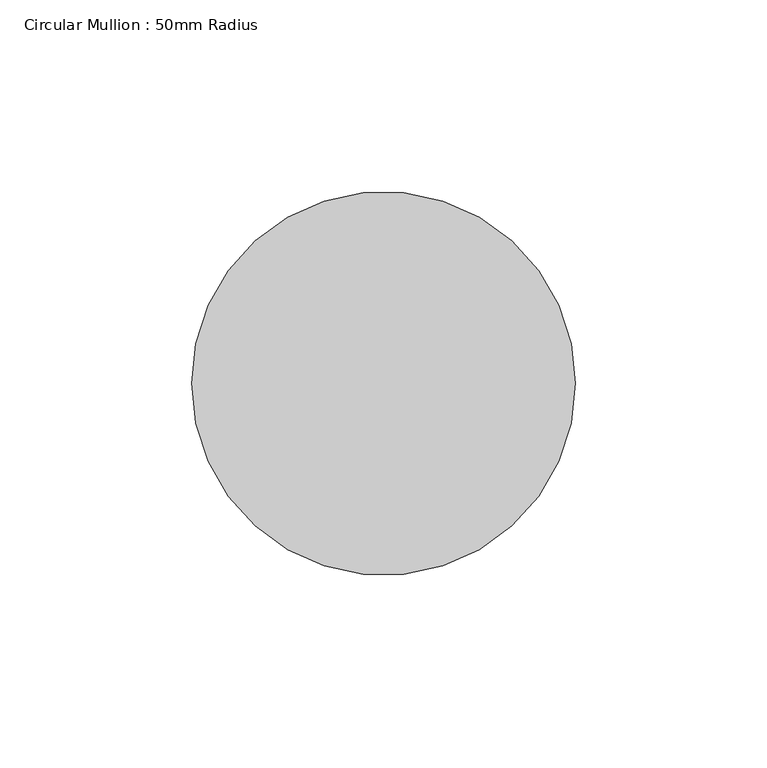
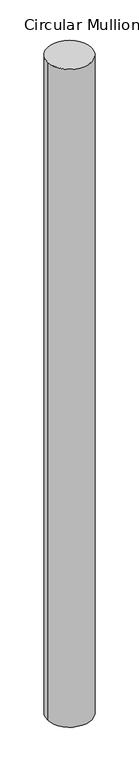
"""IFC4 building model written with IfcOpenShell, lengths in millimetres: member geometry, Circular Mullion : 50mm Radius."""

import ifcopenshell
import ifcopenshell.guid

model = None  # the IFC model being written
_history = None  # IfcOwnerHistory: only IFC2X3 demands one
_inside = {}  # id of a spatial element -> (the spatial element, [elements in it])
_under = {}  # id of a project, library or spatial element -> (it, [spatial elements below it])
_declared = {}  # id of a project -> (the project, [libraries it declares])
_typed = {}  # id of a type object -> (the type object, [elements of that type])
_made_of = {}  # id of a material, layer set ... -> (it, [elements and type objects made of it])


def new_model(schema):
    """Start an empty IFC model of exactly this schema.

    Asked for "IFC4X3", IfcOpenShell would pick the latest addendum, in which some entities
    have other attributes; the version numbers below select the first issue.
    IFC2X3 requires an IfcOwnerHistory on every rooted entity: one is made here for all.
    """
    global model, _history
    if schema == "IFC4X3":
        model = ifcopenshell.file(schema_version=(4, 3, 0, 0))
    else:
        model = ifcopenshell.file(schema=schema)
    _inside.clear()
    _under.clear()
    _declared.clear()
    _typed.clear()
    _made_of.clear()
    _history = None
    if model.schema == "IFC2X3":
        org = make("IfcOrganization", Name="unknown")
        user = make(
            "IfcPersonAndOrganization",
            ThePerson=make("IfcPerson", FamilyName="unknown"),
            TheOrganization=org,
        )
        app = make(
            "IfcApplication",
            ApplicationDeveloper=org,
            Version="unknown",
            ApplicationFullName="unknown",
            ApplicationIdentifier="unknown",
        )
        _history = make(
            "IfcOwnerHistory",
            OwningUser=user,
            OwningApplication=app,
            ChangeAction="ADDED",
            CreationDate=0,
        )
    return model


def make(cls, **values):
    """One entity of the class cls with the attributes given. An attribute that is None is left unset."""
    return model.create_entity(
        cls, **{name: value for name, value in values.items() if value is not None}
    )


def rooted(cls, **values):
    """An entity with a GlobalId (a new one), such as an element, a storey or a relation."""
    return make(cls, GlobalId=ifcopenshell.guid.new(), OwnerHistory=_history, **values)


def si_unit(unit_type, name, prefix=None):
    """IfcSIUnit, for example si_unit("LENGTHUNIT", "METRE", prefix="MILLI")."""
    return make("IfcSIUnit", UnitType=unit_type, Prefix=prefix, Name=name)


def assignment(units):
    """IfcUnitAssignment: the units of a project."""
    return None if units is None else make("IfcUnitAssignment", Units=units)


def point(xyz):
    """IfcCartesianPoint."""
    return None if xyz is None else make("IfcCartesianPoint", Coordinates=xyz)


def direction(xyz):
    """IfcDirection."""
    return None if xyz is None else make("IfcDirection", DirectionRatios=xyz)


def frame(location, z_axis=None, x_axis=None):
    """IfcAxis2Placement3D, a coordinate frame: its origin and axes. An axis left out is left unset."""
    return make(
        "IfcAxis2Placement3D",
        Location=point(location),
        Axis=direction(z_axis),
        RefDirection=direction(x_axis),
    )


def frame_2d(location, x_axis=None):
    """IfcAxis2Placement2D, a coordinate frame in the plane: its origin and x axis."""
    return make(
        "IfcAxis2Placement2D", Location=point(location), RefDirection=direction(x_axis)
    )


def origin():
    """The frame at (0, 0, 0) with its axes left unset."""
    return frame((0.0, 0.0, 0.0))


def origin_2d():
    """The frame at (0, 0) in the plane with its x axis left unset."""
    return frame_2d((0.0, 0.0))


def place(relative_to, where):
    """IfcLocalPlacement: puts the frame where relative to a parent placement (None: the world)."""
    return make(
        "IfcLocalPlacement", PlacementRelTo=relative_to, RelativePlacement=where
    )


def context(
    kind, dimensions, precision=None, world=None, true_north=None, identifier=None
):
    """IfcGeometricRepresentationContext, for example the 3D "Model" context."""
    return make(
        "IfcGeometricRepresentationContext",
        ContextIdentifier=identifier,
        ContextType=kind,
        CoordinateSpaceDimension=dimensions,
        Precision=precision,
        WorldCoordinateSystem=world,
        TrueNorth=true_north,
    )


def project(units=None, contexts=None):
    """IfcProject with its units and contexts."""
    return rooted(
        "IfcProject",
        Name="project",
        RepresentationContexts=contexts,
        UnitsInContext=assignment(units),
    )


def spatial(cls, under=None, at=None, **own):
    """A site, building, storey or space (cls), placed at a placement, below another one or the project."""
    s = rooted(cls, ObjectPlacement=at, **own)
    if under is not None:
        _under.setdefault(under.id(), (under, []))[1].append(s)
    return s


def circle_curve(where, radius):
    """IfcCircle in the frame where."""
    return make("IfcCircle", Position=where, Radius=radius)


def trimmed(basis, trim1, trim2, sense, master):
    """IfcTrimmedCurve: the piece of a basis curve between two trims."""
    return make(
        "IfcTrimmedCurve",
        BasisCurve=basis,
        Trim1=trim1,
        Trim2=trim2,
        SenseAgreement=sense,
        MasterRepresentation=master,
    )


def segment(curve, same_sense, transition):
    """IfcCompositeCurveSegment."""
    return make(
        "IfcCompositeCurveSegment",
        Transition=transition,
        SameSense=same_sense,
        ParentCurve=curve,
    )


def composite_curve(segments, self_intersect=None):
    """IfcCompositeCurve: segments joined end to end."""
    return make("IfcCompositeCurve", Segments=segments, SelfIntersect=self_intersect)


def outline(outer, holes=None, kind="AREA"):
    """IfcArbitraryClosedProfileDef: a profile drawn as a closed curve; with holes, ...WithVoids."""
    if holes is None:
        return make("IfcArbitraryClosedProfileDef", ProfileType=kind, OuterCurve=outer)
    return make(
        "IfcArbitraryProfileDefWithVoids",
        ProfileType=kind,
        OuterCurve=outer,
        InnerCurves=holes,
    )


def extrude(swept, where, along, depth):
    """IfcExtrudedAreaSolid: the profile swept, set in the frame where, extruded along a direction by depth."""
    return make(
        "IfcExtrudedAreaSolid",
        SweptArea=swept,
        Position=where,
        ExtrudedDirection=direction(along),
        Depth=depth,
    )


def shape(context_of_items, identifier, shape_type, items):
    """IfcShapeRepresentation: the items that make up one representation, for example the "Body"."""
    return make(
        "IfcShapeRepresentation",
        ContextOfItems=context_of_items,
        RepresentationIdentifier=identifier,
        RepresentationType=shape_type,
        Items=items,
    )


def source(mapping_origin, context_of_items, identifier, shape_type, items):
    """IfcRepresentationMap: a shape defined once, which mapped items show again and again."""
    return make(
        "IfcRepresentationMap",
        MappingOrigin=mapping_origin,
        MappedRepresentation=shape(context_of_items, identifier, shape_type, items),
    )


def transform(
    local_origin,
    x_axis=None,
    y_axis=None,
    z_axis=None,
    scale=None,
    scale2=None,
    scale3=None,
    uniform=True,
):
    """IfcCartesianTransformationOperator3D, or its non-uniform kind. x_axis, y_axis, z_axis: its Axis1, 2, 3."""
    if uniform:
        return make(
            "IfcCartesianTransformationOperator3D",
            Axis1=direction(x_axis),
            Axis2=direction(y_axis),
            LocalOrigin=point(local_origin),
            Scale=scale,
            Axis3=direction(z_axis),
        )
    return make(
        "IfcCartesianTransformationOperator3DnonUniform",
        Axis1=direction(x_axis),
        Axis2=direction(y_axis),
        LocalOrigin=point(local_origin),
        Scale=scale,
        Axis3=direction(z_axis),
        Scale2=scale2,
        Scale3=scale3,
    )


def mapped(mapping_source, mapping_target):
    """IfcMappedItem: shows the shape of a source again, moved by a transform."""
    return make(
        "IfcMappedItem", MappingSource=mapping_source, MappingTarget=mapping_target
    )


def made_of(thing, what):
    """Note that an element or type object is made of a material, layer set ...; save() writes the relation."""
    if what is not None:
        _made_of.setdefault(what.id(), (what, []))[1].append(thing)
    return thing


def element(
    cls,
    number,
    at=None,
    inside=None,
    cuts=None,
    type_object=None,
    material=None,
    context=None,
    identifier="Body",
    shape_type=None,
    held_by="IfcProductDefinitionShape",
    body=None,
    shapes=None,
    **own,
):
    """One element of the class cls, such as IfcWall. Its Tag is "e" and its number.

    at: its placement. inside: the storey or other place that contains it. cuts: it is an
    opening in that element (IfcRelVoidsElement). A single representation is given by context,
    identifier, shape_type and body (its items); several are given by shapes. held_by: the class
    of the entity that holds the representations. save() writes the other relations.
    """
    e = rooted(cls, Tag="e%d" % number, ObjectPlacement=at, **own)
    if body is not None:
        shapes = [shape(context, identifier, shape_type, body)]
    if shapes is not None:
        e.Representation = make(held_by, Representations=shapes)
    if inside is not None:
        _inside.setdefault(inside.id(), (inside, []))[1].append(e)
    if cuts is not None:
        rooted(
            "IfcRelVoidsElement", RelatingBuildingElement=cuts, RelatedOpeningElement=e
        )
    if type_object is not None:
        _typed.setdefault(type_object.id(), (type_object, []))[1].append(e)
    return made_of(e, material)


def aggregate(whole, parts):
    """IfcRelAggregates: a whole, such as a stair, and the parts it consists of."""
    return rooted("IfcRelAggregates", RelatingObject=whole, RelatedObjects=parts)


def save(model, path):
    """Write the relations noted so far, then the file.

    IfcRelAggregates (storeys below a building ...), IfcRelContainedInSpatialStructure (elements
    in a storey), IfcRelDefinesByType, IfcRelAssociatesMaterial and IfcRelDeclares: one each for
    every whole, place, type object, material and project.
    """
    for whole, parts in _under.values():
        aggregate(whole, parts)
    for where, things in _inside.values():
        rooted(
            "IfcRelContainedInSpatialStructure",
            RelatedElements=things,
            RelatingStructure=where,
        )
    for kind, things in _typed.values():
        rooted("IfcRelDefinesByType", RelatedObjects=things, RelatingType=kind)
    for what, things in _made_of.values():
        rooted("IfcRelAssociatesMaterial", RelatedObjects=things, RelatingMaterial=what)
    for by, libraries in _declared.values():
        rooted("IfcRelDeclares", RelatingContext=by, RelatedDefinitions=libraries)
    model.write(path)


def circular_mullion_50mm_radius_74518a68(model_context):
    return source(origin(), model_context, "Body", "SweptSolid", [
        extrude(outline(composite_curve([segment(trimmed(circle_curve(origin_2d(), 50.0), [point((50.0, 0.0))], [point((-50.0, 0.0))], False, "CARTESIAN"), True, "CONTINUOUS"), segment(trimmed(circle_curve(origin_2d(), 50.0), [point((-50.0, 0.0))], [point((50.0, 0.0))], False, "CARTESIAN"), True, "CONTINUOUS")], self_intersect=False)), frame((0.0, 0.0, -1576.426947), z_axis=(0.0, 0.0, 1.0), x_axis=(1.0, 0.0, 0.0)), (0.0, 0.0, 1.0), 1576.426947),
    ])


if __name__ == "__main__":
    model = new_model("IFC4")
    model_context = context("Model", 3, world=origin())
    ifc_project = project(units=[si_unit("LENGTHUNIT", "METRE", prefix="MILLI")], contexts=[model_context])
    site = spatial("IfcSite", under=ifc_project)
    building = spatial("IfcBuilding", under=site)
    placement = place(None, origin())
    circular_mullion_50mm_radius_shape = circular_mullion_50mm_radius_74518a68(model_context)
    element("IfcMember", 1, ObjectType="Circular Mullion : 50mm Radius", at=placement, inside=building, context=model_context, shape_type="MappedRepresentation", body=[
        mapped(circular_mullion_50mm_radius_shape, transform((0.0, 0.0, 0.0), x_axis=(1.0, 0.0, 0.0), y_axis=(0.0, 1.0, 0.0), z_axis=(0.0, 0.0, 1.0))),
    ])
    save(model, "model.ifc")

# Revit data of these elements
# Type "Circular Mullion : 50mm Radius"
#   built-in parameter 1007350 = 0.164042 (stored number, unit not read)
# Element 1 (IfcMember, "Circular Mullion : 50mm Radius")
#   Materials on its faces: "Aluminium"
# Materials
#   "Aluminium": class "Metal", colour RGB 247 247 247, transparency 0, Description = "Aluminium 6061", Cost = 0
